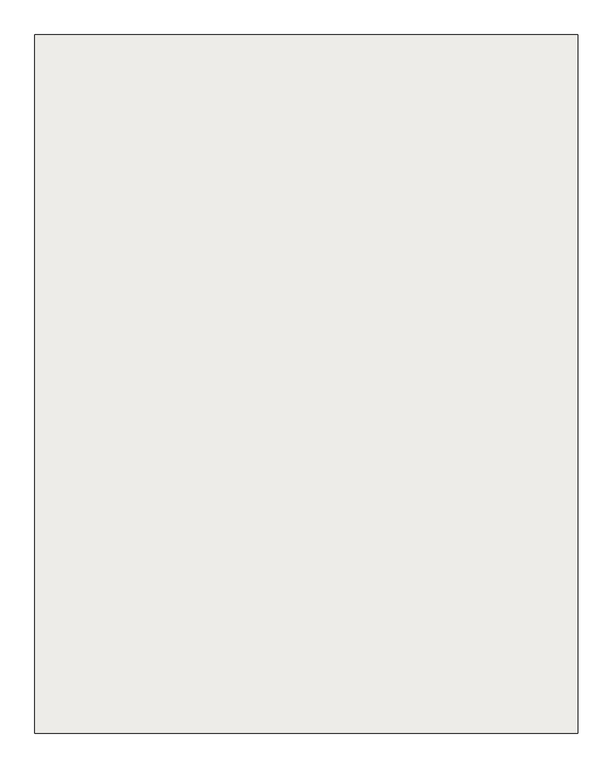
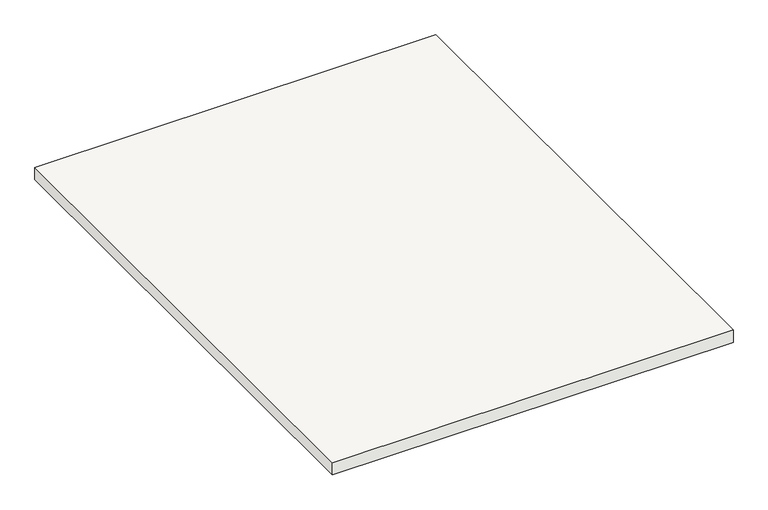
"""IFC4 building model written with IfcOpenShell, lengths in millimetres: slab geometry, Holzdecke 176 : Holzdecke 176."""

from ifc_helpers import new_model, si_unit, frame, origin, place, context, project, spatial, polyline, outline, extrude, source, transform, mapped, element, save


def slab_91406d58(model_context):
    return source(origin(), model_context, "Body", "SweptSolid", [
        extrude(outline(polyline([(15500.0, 19550.0), (15500.0, 1547.1380981), (1500.0, 1547.1380981), (1500.0, 19550.0), (15500.0, 19550.0)])), frame((0.0, 0.0, 2880.0), z_axis=(0.0, 0.0, 1.0), x_axis=(1.0, 0.0, 0.0)), (0.0, 0.0, 1.0), 450.0),
    ])


if __name__ == "__main__":
    model = new_model("IFC4")
    model_context = context("Model", 3, world=origin())
    ifc_project = project(units=[si_unit("LENGTHUNIT", "METRE", prefix="MILLI")], contexts=[model_context])
    site = spatial("IfcSite", under=ifc_project)
    building = spatial("IfcBuilding", under=site)
    placement = place(None, origin())
    slab_shape = slab_91406d58(model_context)
    element("IfcSlab", 1, ObjectType="Holzdecke 176 : Holzdecke 176", at=placement, inside=building, context=model_context, shape_type="MappedRepresentation", body=[
        mapped(slab_shape, transform((0.0, 0.0, 0.0), x_axis=(1.0, 0.0, 0.0), y_axis=(0.0, 1.0, 0.0), z_axis=(0.0, 0.0, 1.0))),
    ])
    save(model, "model.ifc")

# Revit data of these elements
# Type "Holzdecke 176 : Holzdecke 176"
#   Abrechnungsart = "m²"
#   Allright_Bauteil_ID = "0113De 0783954357"
#   Bezeichnung = "Holzdecke"
#   Codetext = "D-HOLZBALKEN1\\"
#   Gewerk = "Zimmer- und Holzbauarbeiten"
#   Material = "Holz"
#   Objektname = "Brettstapeldecke"
#   NameOverride = "Holzdecke"
#   Reference = "Holzdecke"
#   Status = "NEW"
#   PitchAngle = 0.00°
#   ThermalTransmittance = 0.0000 BTU/(h·ft²·°F)
#   2D Interaktion = yes
#   Combustible = no
#   Compartmentation = no
#   IsExternal = no
#   LoadBearing = yes
# Element 1 (IfcSlab, "Holzdecke 176 : Holzdecke 176")
#   Materials on its faces: "holzschalung"
# Materials
#   "holzschalung": class "Unassigned", colour RGB 128 128 128, transparency 0
